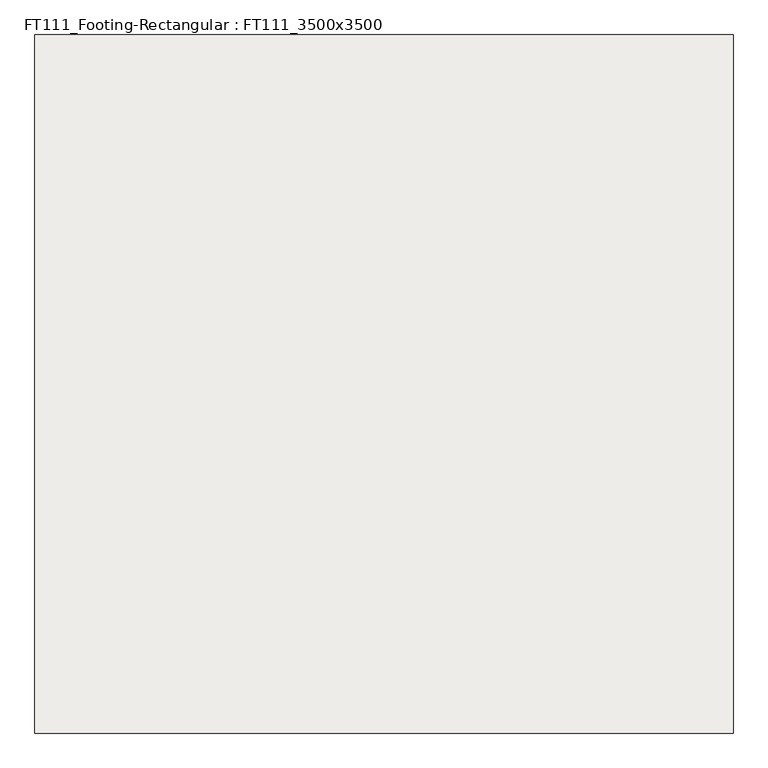
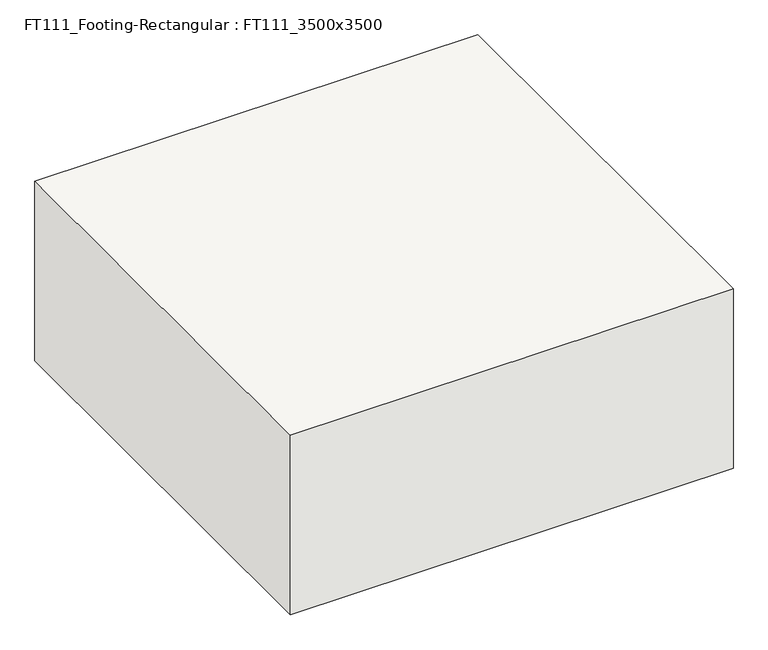
"""IFC4 building model written with IfcOpenShell, lengths in millimetres: slab geometry, FT111_Footing-Rectangular : FT111_3500x3500."""

from ifc_helpers import new_model, si_unit, origin, origin_with_axes, place, context, project, spatial, polyline, outline, extrude, source, transform, mapped, element, save


def ft111_footing_rectangular_ft111_3500x3500_d0491e67(model_context):
    return source(origin(), model_context, "Body", "SweptSolid", [
        extrude(outline(polyline([(1750.0, 1750.0), (1750.0, -1750.0), (-1750.0, -1750.0), (-1750.0, 1750.0), (1750.0, 1750.0)])), origin_with_axes(), (0.0, 0.0, 1.0), 1500.0),
    ])


if __name__ == "__main__":
    model = new_model("IFC4")
    model_context = context("Model", 3, world=origin())
    ifc_project = project(units=[si_unit("LENGTHUNIT", "METRE", prefix="MILLI")], contexts=[model_context])
    site = spatial("IfcSite", under=ifc_project)
    building = spatial("IfcBuilding", under=site)
    placement = place(None, origin())
    ft111_footing_rectangular_ft111_3500x3500_shape = ft111_footing_rectangular_ft111_3500x3500_d0491e67(model_context)
    element("IfcSlab", 1, ObjectType="FT111_Footing-Rectangular : FT111_3500x3500", at=placement, inside=building, context=model_context, shape_type="MappedRepresentation", body=[
        mapped(ft111_footing_rectangular_ft111_3500x3500_shape, transform((0.0, 0.0, 0.0), x_axis=(1.0, 0.0, 0.0), y_axis=(0.0, 1.0, 0.0), z_axis=(0.0, 0.0, 1.0))),
    ])
    save(model, "model.ifc")

# Revit data of these elements
# Type "FT111_Footing-Rectangular : FT111_3500x3500"
#   Assembly Code = "A1010100"
#   Width = 3500 mm
#   Length = 3500 mm
#   Foundation Thickness = 1500 mm
#   Structural Material [instance default] = Concrete, Cast-in-Place gray
# Element 1 (IfcSlab, "FT111_Footing-Rectangular : FT111_3500x3500")
#   Materials on its faces: "Concrete, Cast-in-Place gray"
# Materials
#   "Concrete, Cast-in-Place gray": class "Concrete", colour RGB 192 192 192, transparency 0, Description = "Cast-in-place concrete", Cost = 0
